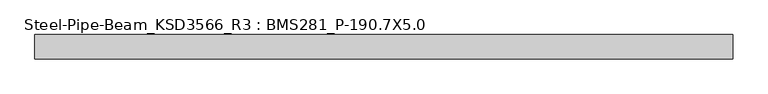
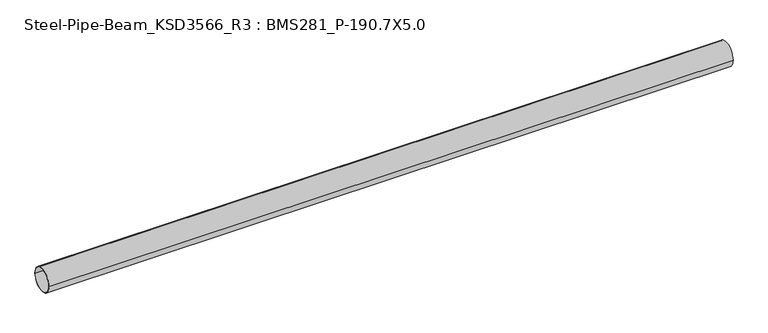
"""IFC4 building model written with IfcOpenShell, lengths in millimetres: member geometry, Steel-Pipe-Beam_KSD3566_R3 : BMS281_P-190.7X5.0."""

from ifc_helpers import new_model, si_unit, point, frame, origin, origin_2d, place, context, project, spatial, circle_curve, trimmed, segment, composite_curve, outline, extrude, source, transform, mapped, element, save


def steel_pipe_beam_ksd3566_r3_bms281_p_190_7x5_0_090b0653(model_context):
    return source(origin(), model_context, "Body", "SweptSolid", [
        extrude(outline(composite_curve([segment(trimmed(circle_curve(origin_2d(), 95.35), [point((-95.35, 0.0))], [point((95.35, 0.0))], False, "CARTESIAN"), True, "CONTINUOUS"), segment(trimmed(circle_curve(origin_2d(), 95.35), [point((95.35, 0.0))], [point((-95.35, 0.0))], False, "CARTESIAN"), True, "CONTINUOUS")], self_intersect=False), holes=[composite_curve([segment(trimmed(circle_curve(origin_2d(), 90.35), [point((90.35, 0.0))], [point((-90.35, 0.0))], True, "CARTESIAN"), True, "CONTINUOUS"), segment(trimmed(circle_curve(origin_2d(), 90.35), [point((-90.35, 0.0))], [point((90.35, 0.0))], True, "CARTESIAN"), True, "CONTINUOUS")], self_intersect=False)]), frame((-2674.7801619, 0.0, 0.0), z_axis=(1.0, 0.0, 0.0), x_axis=(0.0, 1.0, 0.0)), (0.0, 0.0, 1.0), 5417.7988461),
    ])


if __name__ == "__main__":
    model = new_model("IFC4")
    model_context = context("Model", 3, world=origin())
    ifc_project = project(units=[si_unit("LENGTHUNIT", "METRE", prefix="MILLI")], contexts=[model_context])
    site = spatial("IfcSite", under=ifc_project)
    building = spatial("IfcBuilding", under=site)
    placement = place(None, origin())
    steel_pipe_beam_ksd3566_r3_bms281_p_190_7x5_0_shape = steel_pipe_beam_ksd3566_r3_bms281_p_190_7x5_0_090b0653(model_context)
    element("IfcMember", 1, ObjectType="Steel-Pipe-Beam_KSD3566_R3 : BMS281_P-190.7X5.0", at=placement, inside=building, context=model_context, shape_type="MappedRepresentation", body=[
        mapped(steel_pipe_beam_ksd3566_r3_bms281_p_190_7x5_0_shape, transform((0.0, 0.0, 0.0), x_axis=(1.0, 0.0, 0.0), y_axis=(0.0, 1.0, 0.0), z_axis=(0.0, 0.0, 1.0))),
    ])
    save(model, "model.ifc")

# Revit data of these elements
# Type "Steel-Pipe-Beam_KSD3566_R3 : BMS281_P-190.7X5.0"
#   Keynote = "P-190.7X5.0"
#   SteelWeight = "Light"
#   t = 0.0050 m
#   Surface Area = 0.599102 m²/m
#   Section Area = 29.1697 cm²
#   Mass per Unit Length = 22.8982 kg/m
#   Length [instance default] = 1.5000 m
#   D = 0.1907 m
#   hec_material4 [instance default] = none
#   hec_material3 [instance default] = none
#   hec_material2 [instance default] = none
#   hec_material1 [instance default] = none
#   Structural Material [instance default] = Steel, 45-345
#   Assembly Code = ""
# Element 1 (IfcMember, "Steel-Pipe-Beam_KSD3566_R3 : BMS281_P-190.7X5.0")
#   Structural Material = none
# Materials
#   "Steel, 45-345": class "Metal", colour RGB 189 187 185, transparency 0, Description = "Steel 345 MPa", Cost = 0
